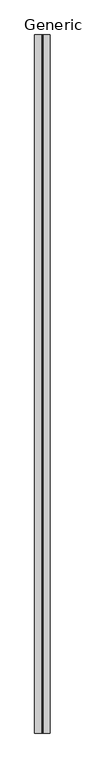
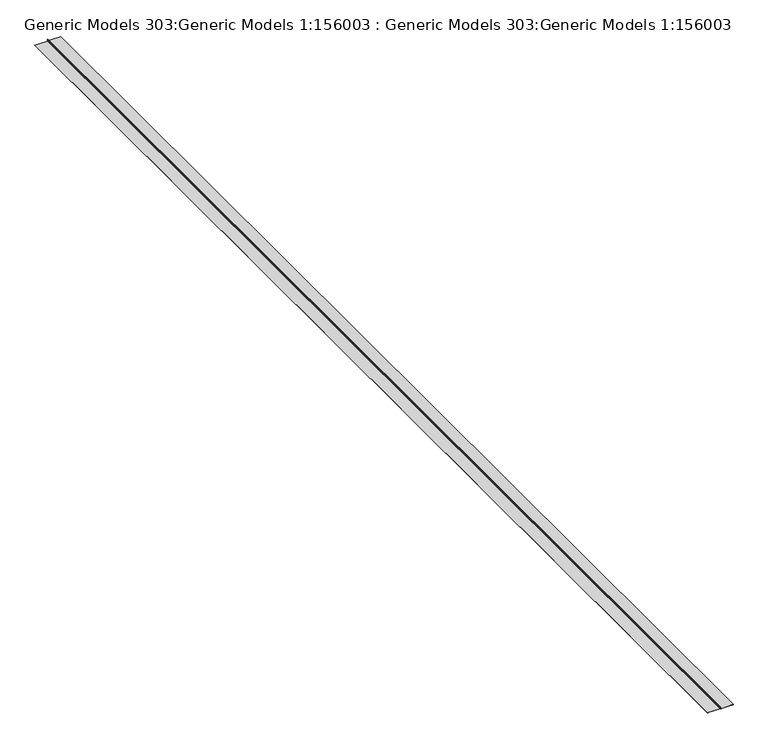
"""IFC4 building model written with IfcOpenShell, lengths in millimetres: proxy geometry, Generic Models 303:Generic Models 1:156003 : Generic Models 303:Generic Models 1:156003."""

from ifc_helpers import new_model, si_unit, point, frame, frame_2d, origin, place, context, project, spatial, polyline, circle_curve, trimmed, segment, composite_curve, outline, extrude, source, transform, mapped, element, save
from ifc_brep_helpers import plane_surface, cylinder_surface, revolved_surface, advanced_brep


def generic_models_303_generic_models_1_156003_generic_models_23746147(model_context):
    return source(origin(), model_context, "Body", "SolidModel", [
        extrude(outline(composite_curve([segment(polyline([(6881.3731364, -6977.9100218), (6882.16353, -6977.9100218)]), True, "CONTINUOUS"), segment(trimmed(circle_curve(frame_2d((6884.9227743, -6977.9100218)), 2.7592444), [point((6882.16353, -6977.9100218))], [point((6885.9425422, -6980.4739062))], True, "CARTESIAN"), True, "CONTINUOUS"), segment(polyline([(6885.9425422, -6980.4739062), (6895.9865066, -6976.4789867)]), True, "CONTINUOUS"), segment(trimmed(circle_curve(frame_2d((6894.8331732, -6974.1073382)), 2.6372134), [point((6895.9865066, -6976.4789867))], [point((6896.038172, -6971.761518))], True, "CARTESIAN"), True, "CONTINUOUS"), segment(trimmed(circle_curve(frame_2d((6874.6910483, -7052.7950767)), 83.798194), [point((6896.038172, -6971.761518))], [point((6884.6021494, -6969.5850569))], True, "CARTESIAN"), True, "CONTINUOUS"), segment(trimmed(circle_curve(frame_2d((6884.2734301, -6971.2056712)), 1.6536163), [point((6884.6021494, -6969.5850569))], [point((6882.7768168, -6970.5023964))], True, "CARTESIAN"), True, "CONTINUOUS"), segment(trimmed(circle_curve(frame_2d((6881.47319, -6969.8955806)), 1.4379388), [point((6882.7768168, -6970.5023964))], [point((6881.4500793, -6971.3333337))], False, "CARTESIAN"), True, "CONTINUOUS"), segment(polyline([(6881.4500793, -6971.3333337), (6866.1481908, -6971.0662383), (6864.7043721, -6764.5647547), (6865.5795866, -6764.5647547), (6867.0179843, -6970.2909066), (6881.9187348, -6970.5510002)]), True, "CONTINUOUS"), segment(trimmed(circle_curve(frame_2d((6884.2734301, -6971.2056712)), 2.4440099), [point((6881.9187348, -6970.5510002))], [point((6884.7246111, -6968.8036679))], False, "CARTESIAN"), True, "CONTINUOUS"), segment(trimmed(circle_curve(frame_2d((6874.6910483, -7052.7950767)), 84.5885876), [point((6884.7246111, -6968.8036679))], [point((6896.3174348, -6971.017766))], False, "CARTESIAN"), True, "CONTINUOUS"), segment(trimmed(circle_curve(frame_2d((6894.8331732, -6974.1073382)), 3.4276069), [point((6896.3174348, -6971.017766))], [point((6896.3040507, -6977.2033047))], False, "CARTESIAN"), True, "CONTINUOUS"), segment(polyline([(6896.3040507, -6977.2033047), (6886.2346576, -6981.2083383)]), True, "CONTINUOUS"), segment(trimmed(circle_curve(frame_2d((6884.9227743, -6977.9100218)), 3.5496379), [point((6886.2346576, -6981.2083383))], [point((6881.3731364, -6977.9100218))], False, "CARTESIAN"), True, "CONTINUOUS")], self_intersect=False)), frame((0.0, -19323.9974793, 0.0), z_axis=(0.0, 1.0, 0.0), x_axis=(0.0, 0.0, 1.0)), (0.0, 0.0, 1.0), 19050.0),
        extrude(outline(composite_curve([segment(trimmed(circle_curve(frame_2d((6892.8380638, -6973.8225733)), 2.2809286), [point((6893.6721873, -6971.6996335))], [point((6894.0377051, -6975.7625466))], False, "CARTESIAN"), True, "CONTINUOUS"), segment(trimmed(circle_curve(frame_2d((6918.3848934, -7036.3176657)), 65.2664388), [point((6894.0377051, -6975.7625466))], [point((6889.5431069, -6977.7697419))], True, "CARTESIAN"), True, "CONTINUOUS"), segment(polyline([(6889.5431069, -6977.7697419), (6889.1888233, -6977.0517094)]), True, "CONTINUOUS"), segment(trimmed(circle_curve(frame_2d((6918.1556369, -7035.7592364)), 65.4648763), [point((6889.1888233, -6977.0517094))], [point((6893.7182187, -6975.0265219))], False, "CARTESIAN"), True, "CONTINUOUS"), segment(trimmed(circle_curve(frame_2d((6893.0001599, -6973.7976617)), 1.4232729), [point((6893.7182187, -6975.0265219))], [point((6893.5621185, -6972.4900271))], True, "CARTESIAN"), True, "CONTINUOUS"), segment(polyline([(6893.5621185, -6972.4900271), (6863.2388437, -6972.4900271), (6863.2388437, -6960.4209665), (6864.7321656, -6958.9276446), (6864.7321656, -6955.3836986), (6863.5982917, -6954.2313379), (6863.5982917, -6953.1349596), (6865.5225591, -6955.0798395), (6865.5225591, -6959.2321209), (6864.0292373, -6960.7254427), (6864.0292373, -6971.6996335), (6893.6721873, -6971.6996335)]), True, "CONTINUOUS")], self_intersect=False)), frame((0.0, -19323.9974793, 0.0), z_axis=(0.0, 1.0, 0.0), x_axis=(0.0, 0.0, 1.0)), (0.0, 0.0, 1.0), 19050.0),
        advanced_brep(
        [(-6974.8109562, -273.9974793, 6864.1193209), (-6973.6115547, -273.9974793, 6891.5901334), (-6974.6776604, -273.9974793, 6891.8032811), (-6978.558406, -273.9974793, 6883.177829), (-6979.2527572, -273.9974793, 6883.5522549), (-6975.4226513, -273.9974793, 6892.0673609), (-6972.8219134, -273.9974793, 6891.5556569), (-6974.0582522, -273.9974793, 6863.2388437), (-7183.6647547, -273.9974793, 6864.7043721), (-7183.6647547, -273.9974793, 6865.5795866), (-6974.8109562, -19323.9974793, 6864.1193209), (-7183.6647547, -19323.9974793, 6865.5795866), (-7183.6647547, -19323.9974793, 6864.7043721), (-6974.0582522, -19323.9974793, 6863.2388437), (-6972.8219134, -19323.9974793, 6891.5556569), (-6975.4226513, -19323.9974793, 6892.0673609), (-6979.2527572, -19323.9974793, 6883.5522549), (-6978.558406, -19323.9974793, 6883.177829), (-6974.676296, -19323.9974793, 6891.8069663), (-6973.6115547, -19323.9974793, 6891.5901334)],
        [
            (0, 1),
            (1, 2, circle_curve(frame((-6974.1611177, -273.9974793, 6891.6141278), z_axis=(0.0, -1.0, 0.0), x_axis=(1.0, 0.0, 0.0)), 0.5500866)),
            (2, 3, circle_curve(frame((-7036.6125559, -273.9974793, 6914.4832755), z_axis=(0.0, 1.0, 0.0), x_axis=(1.0, 0.0, 0.0)), 65.9569199)),
            (3, 4),
            (4, 5, circle_curve(frame((-7036.8889703, -273.9974793, 6914.596046), z_axis=(0.0, -1.0, 0.0), x_axis=(1.0, 0.0, 0.0)), 65.4648763)),
            (5, 6, circle_curve(frame((-6974.1748164, -273.9974793, 6891.5445042), z_axis=(0.0, 1.0, 0.0), x_axis=(1.0, 0.0, 0.0)), 1.352949)),
            (6, 7),
            (7, 8),
            (8, 9),
            (9, 0),
            (10, 11),
            (11, 12),
            (12, 13),
            (13, 14),
            (14, 15, circle_curve(frame((-6974.1748164, -19323.9974793, 6891.5445042), z_axis=(0.0, -1.0, 0.0), x_axis=(1.0, 0.0, 0.0)), 1.352949)),
            (15, 16, circle_curve(frame((-7036.8889703, -19323.9974793, 6914.596046), z_axis=(0.0, 1.0, 0.0), x_axis=(1.0, 0.0, 0.0)), 65.4648763)),
            (16, 17),
            (17, 18, circle_curve(frame((-7036.6125559, -19323.9974793, 6914.4832755), z_axis=(0.0, -1.0, 0.0), x_axis=(1.0, 0.0, 0.0)), 65.9569199)),
            (18, 19, circle_curve(frame((-6974.1611177, -19323.9974793, 6891.6141278), z_axis=(0.0, 1.0, 0.0), x_axis=(1.0, 0.0, 0.0)), 0.5500866)),
            (19, 10),
            (0, 10),
            (19, 1),
            (18, 2),
            (17, 3),
            (16, 4),
            (15, 5),
            (14, 6),
            (13, 7),
            (12, 8),
            (11, 9),
        ],
        [
            plane_surface(frame((-6973.6115547, -273.9974793, 6891.5901334), z_axis=(0.0, 1.0, 0.0), x_axis=(0.043619387365286685, 0.0, 0.9990482215818599))),
            plane_surface(frame((-6973.6115547, -19323.9974793, 6891.5901334), z_axis=(0.0, -1.0, 0.0), x_axis=(-0.043619387365286685, 0.0, -0.9990482215818599))),
            plane_surface(frame((-6974.8109562, -273.9974793, 6864.1193209), z_axis=(-0.9990482215818599, 0.0, 0.043619387365286685), x_axis=(0.0, -1.0, 0.0))),
            revolved_surface(polyline([(-6973.6110311, -19323.9974793, 6891.6141278), (-6973.6110311, -273.9974793000001, 6891.6141278)]), (-6974.1611177, -19323.9974793, 6891.6141278), (0.0, -1.0, 0.0)),
            cylinder_surface(frame((-7036.6125559, -19323.9974793, 6914.4832755), z_axis=(0.0, 1.0, 0.0), x_axis=(1.0, 0.0, 0.0)), 65.9569199),
            plane_surface(frame((-6978.558406, -273.9974793, 6883.177829), z_axis=(-0.474634753614868, 0.0, -0.8801828506969183), x_axis=(0.0, -1.0, 0.0))),
            revolved_surface(polyline([(-6971.424094000001, -19323.9974793, 6914.596046), (-6971.424094000001, -273.9974793000001, 6914.596046)]), (-7036.8889703, -19323.9974793, 6914.596046), (0.0, -1.0, 0.0)),
            cylinder_surface(frame((-6974.1748164, -19323.9974793, 6891.5445042), z_axis=(0.0, 1.0, 0.0), x_axis=(1.0, 0.0, 0.0)), 1.352949),
            plane_surface(frame((-6972.8219134, -273.9974793, 6891.5556569), z_axis=(0.9990482215818648, 0.0, -0.043619387365175705), x_axis=(0.0, -1.0, 0.0))),
            plane_surface(frame((-6974.0582522, -273.9974793, 6863.2388437), z_axis=(-0.00699163697333996, 0.0, -0.9999755582075159), x_axis=(0.0, -1.0, 0.0))),
            plane_surface(frame((-7183.6647547, -273.9974793, 6864.7043721), z_axis=(-1.0, 0.0, 0.0), x_axis=(0.0, -1.0, 0.0))),
            plane_surface(frame((-7183.6647547, -273.9974793, 6865.5795866), z_axis=(0.006991636973340252, 0.0, 0.9999755582075159), x_axis=(0.0, -1.0, 0.0))),
        ],
        [
            (0, [[1, 2, 3, 4, 5, 6, 7, 8, 9, 10]]),
            (1, [[11, 12, 13, 14, 15, 16, 17, 18, 19, 20]]),
            (2, [[-1, 21, -20, 22]]),
            (3, [[-2, -22, -19, 23]]),
            (4, [[-3, -23, -18, 24]]),
            (5, [[-4, -24, -17, 25]]),
            (6, [[-5, -25, -16, 26]]),
            (7, [[-6, -26, -15, 27]]),
            (8, [[-7, -27, -14, 28]]),
            (9, [[-8, -28, -13, 29]]),
            (10, [[-9, -29, -12, 30]]),
            (11, [[-10, -30, -11, -21]]),
        ],
    ),
    ])


if __name__ == "__main__":
    model = new_model("IFC4")
    model_context = context("Model", 3, world=origin())
    ifc_project = project(units=[si_unit("LENGTHUNIT", "METRE", prefix="MILLI")], contexts=[model_context])
    site = spatial("IfcSite", under=ifc_project)
    building = spatial("IfcBuilding", under=site)
    placement = place(None, origin())
    generic_models_303_generic_models_1_156003_generic_models_shape = generic_models_303_generic_models_1_156003_generic_models_23746147(model_context)
    element("IfcBuildingElementProxy", 1, Name="Generic Models 303:Generic Models 1:156003 : Generic Models 303:Generic Models 1:156003", ObjectType="Generic Models 303:Generic Models 1:156003 : Generic Models 303:Generic Models 1:156003", at=placement, inside=building, context=model_context, shape_type="MappedRepresentation", body=[
        mapped(generic_models_303_generic_models_1_156003_generic_models_shape, transform((0.0, 0.0, 0.0), x_axis=(1.0, 0.0, 0.0), y_axis=(0.0, 1.0, 0.0), z_axis=(0.0, 0.0, 1.0))),
    ])
    save(model, "model.ifc")

# Revit data of these elements
# Type "Generic Models 303:Generic Models 1:156003 : Generic Models 303:Generic Models 1:156003"
#   NameOverride = "Generic Models 303:Generic Models 1:156003"
#   ObjectTypeOverride = "Generic Models 303:Generic Models 1"
#   Reference = "Generic Models 1"
#   Category = "Generic Models"
#   Tag = "156003"
# Element 1 (IfcBuildingElementProxy, "Generic Models 303:Generic Models 1:156003 : Generic Models 303:Generic Models 1:156003")
#   Materials on its faces: "_STANDING SEAM METAL ROOF PER SPECS 36954"
# Materials
#   "_STANDING SEAM METAL ROOF PER SPECS 36954": class "Unassigned", colour RGB 175 175 175, transparency 0
